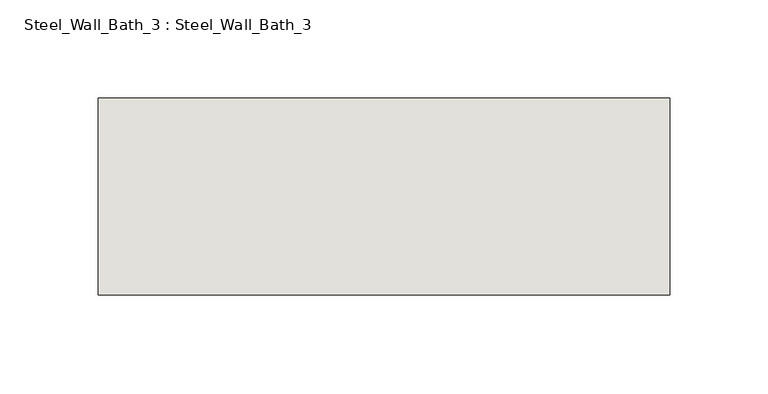
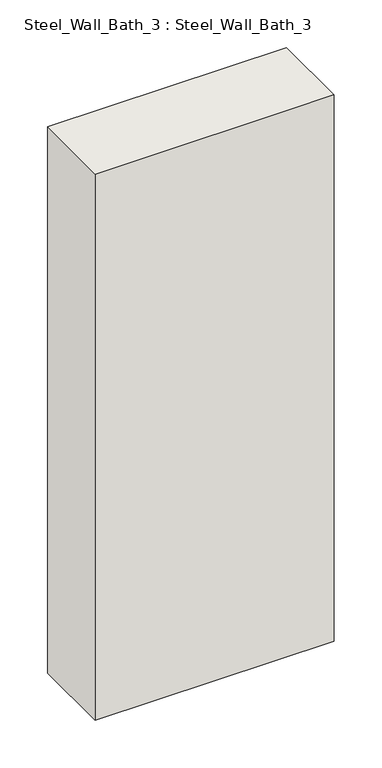
"""IFC4 building model written with IfcOpenShell, lengths in millimetres: wall geometry, Steel_Wall_Bath_3 : Steel_Wall_Bath_3."""

import ifcopenshell
import ifcopenshell.guid

model = None  # the IFC model being written
_history = None  # IfcOwnerHistory: only IFC2X3 demands one
_inside = {}  # id of a spatial element -> (the spatial element, [elements in it])
_under = {}  # id of a project, library or spatial element -> (it, [spatial elements below it])
_declared = {}  # id of a project -> (the project, [libraries it declares])
_typed = {}  # id of a type object -> (the type object, [elements of that type])
_made_of = {}  # id of a material, layer set ... -> (it, [elements and type objects made of it])


def new_model(schema):
    """Start an empty IFC model of exactly this schema.

    Asked for "IFC4X3", IfcOpenShell would pick the latest addendum, in which some entities
    have other attributes; the version numbers below select the first issue.
    IFC2X3 requires an IfcOwnerHistory on every rooted entity: one is made here for all.
    """
    global model, _history
    if schema == "IFC4X3":
        model = ifcopenshell.file(schema_version=(4, 3, 0, 0))
    else:
        model = ifcopenshell.file(schema=schema)
    _inside.clear()
    _under.clear()
    _declared.clear()
    _typed.clear()
    _made_of.clear()
    _history = None
    if model.schema == "IFC2X3":
        org = make("IfcOrganization", Name="unknown")
        user = make(
            "IfcPersonAndOrganization",
            ThePerson=make("IfcPerson", FamilyName="unknown"),
            TheOrganization=org,
        )
        app = make(
            "IfcApplication",
            ApplicationDeveloper=org,
            Version="unknown",
            ApplicationFullName="unknown",
            ApplicationIdentifier="unknown",
        )
        _history = make(
            "IfcOwnerHistory",
            OwningUser=user,
            OwningApplication=app,
            ChangeAction="ADDED",
            CreationDate=0,
        )
    return model


def make(cls, **values):
    """One entity of the class cls with the attributes given. An attribute that is None is left unset."""
    return model.create_entity(
        cls, **{name: value for name, value in values.items() if value is not None}
    )


def rooted(cls, **values):
    """An entity with a GlobalId (a new one), such as an element, a storey or a relation."""
    return make(cls, GlobalId=ifcopenshell.guid.new(), OwnerHistory=_history, **values)


def si_unit(unit_type, name, prefix=None):
    """IfcSIUnit, for example si_unit("LENGTHUNIT", "METRE", prefix="MILLI")."""
    return make("IfcSIUnit", UnitType=unit_type, Prefix=prefix, Name=name)


def assignment(units):
    """IfcUnitAssignment: the units of a project."""
    return None if units is None else make("IfcUnitAssignment", Units=units)


def point(xyz):
    """IfcCartesianPoint."""
    return None if xyz is None else make("IfcCartesianPoint", Coordinates=xyz)


def direction(xyz):
    """IfcDirection."""
    return None if xyz is None else make("IfcDirection", DirectionRatios=xyz)


def frame(location, z_axis=None, x_axis=None):
    """IfcAxis2Placement3D, a coordinate frame: its origin and axes. An axis left out is left unset."""
    return make(
        "IfcAxis2Placement3D",
        Location=point(location),
        Axis=direction(z_axis),
        RefDirection=direction(x_axis),
    )


def origin():
    """The frame at (0, 0, 0) with its axes left unset."""
    return frame((0.0, 0.0, 0.0))


def place(relative_to, where):
    """IfcLocalPlacement: puts the frame where relative to a parent placement (None: the world)."""
    return make(
        "IfcLocalPlacement", PlacementRelTo=relative_to, RelativePlacement=where
    )


def context(
    kind, dimensions, precision=None, world=None, true_north=None, identifier=None
):
    """IfcGeometricRepresentationContext, for example the 3D "Model" context."""
    return make(
        "IfcGeometricRepresentationContext",
        ContextIdentifier=identifier,
        ContextType=kind,
        CoordinateSpaceDimension=dimensions,
        Precision=precision,
        WorldCoordinateSystem=world,
        TrueNorth=true_north,
    )


def project(units=None, contexts=None):
    """IfcProject with its units and contexts."""
    return rooted(
        "IfcProject",
        Name="project",
        RepresentationContexts=contexts,
        UnitsInContext=assignment(units),
    )


def spatial(cls, under=None, at=None, **own):
    """A site, building, storey or space (cls), placed at a placement, below another one or the project."""
    s = rooted(cls, ObjectPlacement=at, **own)
    if under is not None:
        _under.setdefault(under.id(), (under, []))[1].append(s)
    return s


def polyline(points):
    """IfcPolyline through the points."""
    return make("IfcPolyline", Points=[point(p) for p in points])


def outline(outer, holes=None, kind="AREA"):
    """IfcArbitraryClosedProfileDef: a profile drawn as a closed curve; with holes, ...WithVoids."""
    if holes is None:
        return make("IfcArbitraryClosedProfileDef", ProfileType=kind, OuterCurve=outer)
    return make(
        "IfcArbitraryProfileDefWithVoids",
        ProfileType=kind,
        OuterCurve=outer,
        InnerCurves=holes,
    )


def extrude(swept, where, along, depth):
    """IfcExtrudedAreaSolid: the profile swept, set in the frame where, extruded along a direction by depth."""
    return make(
        "IfcExtrudedAreaSolid",
        SweptArea=swept,
        Position=where,
        ExtrudedDirection=direction(along),
        Depth=depth,
    )


def shape(context_of_items, identifier, shape_type, items):
    """IfcShapeRepresentation: the items that make up one representation, for example the "Body"."""
    return make(
        "IfcShapeRepresentation",
        ContextOfItems=context_of_items,
        RepresentationIdentifier=identifier,
        RepresentationType=shape_type,
        Items=items,
    )


def source(mapping_origin, context_of_items, identifier, shape_type, items):
    """IfcRepresentationMap: a shape defined once, which mapped items show again and again."""
    return make(
        "IfcRepresentationMap",
        MappingOrigin=mapping_origin,
        MappedRepresentation=shape(context_of_items, identifier, shape_type, items),
    )


def transform(
    local_origin,
    x_axis=None,
    y_axis=None,
    z_axis=None,
    scale=None,
    scale2=None,
    scale3=None,
    uniform=True,
):
    """IfcCartesianTransformationOperator3D, or its non-uniform kind. x_axis, y_axis, z_axis: its Axis1, 2, 3."""
    if uniform:
        return make(
            "IfcCartesianTransformationOperator3D",
            Axis1=direction(x_axis),
            Axis2=direction(y_axis),
            LocalOrigin=point(local_origin),
            Scale=scale,
            Axis3=direction(z_axis),
        )
    return make(
        "IfcCartesianTransformationOperator3DnonUniform",
        Axis1=direction(x_axis),
        Axis2=direction(y_axis),
        LocalOrigin=point(local_origin),
        Scale=scale,
        Axis3=direction(z_axis),
        Scale2=scale2,
        Scale3=scale3,
    )


def mapped(mapping_source, mapping_target):
    """IfcMappedItem: shows the shape of a source again, moved by a transform."""
    return make(
        "IfcMappedItem", MappingSource=mapping_source, MappingTarget=mapping_target
    )


def made_of(thing, what):
    """Note that an element or type object is made of a material, layer set ...; save() writes the relation."""
    if what is not None:
        _made_of.setdefault(what.id(), (what, []))[1].append(thing)
    return thing


def element(
    cls,
    number,
    at=None,
    inside=None,
    cuts=None,
    type_object=None,
    material=None,
    context=None,
    identifier="Body",
    shape_type=None,
    held_by="IfcProductDefinitionShape",
    body=None,
    shapes=None,
    **own,
):
    """One element of the class cls, such as IfcWall. Its Tag is "e" and its number.

    at: its placement. inside: the storey or other place that contains it. cuts: it is an
    opening in that element (IfcRelVoidsElement). A single representation is given by context,
    identifier, shape_type and body (its items); several are given by shapes. held_by: the class
    of the entity that holds the representations. save() writes the other relations.
    """
    e = rooted(cls, Tag="e%d" % number, ObjectPlacement=at, **own)
    if body is not None:
        shapes = [shape(context, identifier, shape_type, body)]
    if shapes is not None:
        e.Representation = make(held_by, Representations=shapes)
    if inside is not None:
        _inside.setdefault(inside.id(), (inside, []))[1].append(e)
    if cuts is not None:
        rooted(
            "IfcRelVoidsElement", RelatingBuildingElement=cuts, RelatedOpeningElement=e
        )
    if type_object is not None:
        _typed.setdefault(type_object.id(), (type_object, []))[1].append(e)
    return made_of(e, material)


def aggregate(whole, parts):
    """IfcRelAggregates: a whole, such as a stair, and the parts it consists of."""
    return rooted("IfcRelAggregates", RelatingObject=whole, RelatedObjects=parts)


def save(model, path):
    """Write the relations noted so far, then the file.

    IfcRelAggregates (storeys below a building ...), IfcRelContainedInSpatialStructure (elements
    in a storey), IfcRelDefinesByType, IfcRelAssociatesMaterial and IfcRelDeclares: one each for
    every whole, place, type object, material and project.
    """
    for whole, parts in _under.values():
        aggregate(whole, parts)
    for where, things in _inside.values():
        rooted(
            "IfcRelContainedInSpatialStructure",
            RelatedElements=things,
            RelatingStructure=where,
        )
    for kind, things in _typed.values():
        rooted("IfcRelDefinesByType", RelatedObjects=things, RelatingType=kind)
    for what, things in _made_of.values():
        rooted("IfcRelAssociatesMaterial", RelatedObjects=things, RelatingMaterial=what)
    for by, libraries in _declared.values():
        rooted("IfcRelDeclares", RelatingContext=by, RelatedDefinitions=libraries)
    model.write(path)


def steel_wall_bath_3_steel_wall_bath_3_592d521f(model_context):
    return source(origin(), model_context, "Body", "SweptSolid", [
        extrude(outline(polyline([(4365.0, 12105.0), (4075.0, 12105.0), (4075.0, 12205.0), (4365.0, 12205.0), (4365.0, 12105.0)])), frame((0.0, 0.0, 2850.0), z_axis=(0.0, 0.0, 1.0), x_axis=(1.0, 0.0, 0.0)), (0.0, 0.0, 1.0), 700.0),
    ])


if __name__ == "__main__":
    model = new_model("IFC4")
    model_context = context("Model", 3, world=origin())
    ifc_project = project(units=[si_unit("LENGTHUNIT", "METRE", prefix="MILLI")], contexts=[model_context])
    site = spatial("IfcSite", under=ifc_project)
    building = spatial("IfcBuilding", under=site)
    placement = place(None, origin())
    steel_wall_bath_3_steel_wall_bath_3_shape = steel_wall_bath_3_steel_wall_bath_3_592d521f(model_context)
    element("IfcWall", 1, ObjectType="Steel_Wall_Bath_3 : Steel_Wall_Bath_3", at=placement, inside=building, context=model_context, shape_type="MappedRepresentation", body=[
        mapped(steel_wall_bath_3_steel_wall_bath_3_shape, transform((0.0, 0.0, 0.0), x_axis=(1.0, 0.0, 0.0), y_axis=(0.0, 1.0, 0.0), z_axis=(0.0, 0.0, 1.0))),
    ])
    save(model, "model.ifc")

# Revit data of these elements
# Type "Steel_Wall_Bath_3 : Steel_Wall_Bath_3"
#   NameOverride = "Steel_Wall_Bath_3"
# Element 1 (IfcWall, "Steel_Wall_Bath_3 : Steel_Wall_Bath_3")
#   Materials on its faces: "IfcSurfaceStyle #33"
# Materials
#   "IfcSurfaceStyle #33": class "Unassigned", colour RGB 214 214 214, transparency 0
